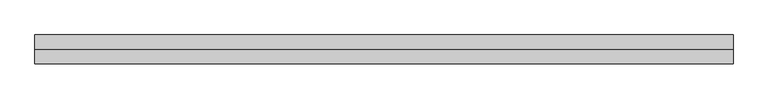
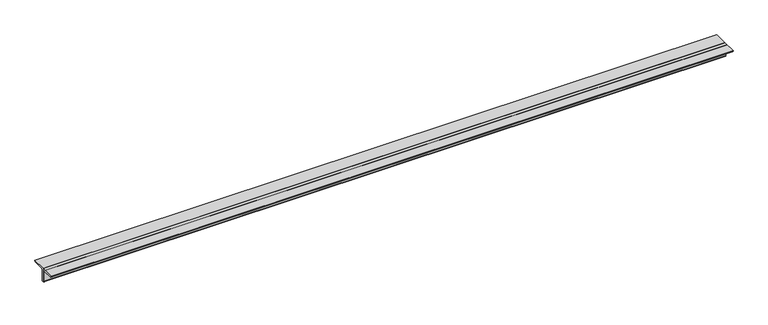
"""IFC4 building model written with IfcOpenShell, lengths in millimetres: member geometry, 0123_Steel Framing_2Ls-KSD3502 : H_SB_AR_S04_2Ls-130x130x12_VBR2."""

from ifc_helpers import new_model, si_unit, point, frame, frame_2d, origin, place, context, project, spatial, polyline, circle_curve, trimmed, segment, composite_curve, outline, extrude, source, transform, mapped, element, save


def member_81b2beba(model_context):
    return source(origin(), model_context, "Body", "SweptSolid", [
        extrude(outline(composite_curve([segment(polyline([(0.0, 36.4), (130.0, 36.4)]), True, "CONTINUOUS"), segment(trimmed(circle_curve(frame_2d((118.0, 36.4)), 12.0), [point((130.0, 36.4))], [point((118.0, 24.4))], False, "CARTESIAN"), True, "CONTINUOUS"), segment(polyline([(118.0, 24.4), (24.0, 24.4)]), True, "CONTINUOUS"), segment(trimmed(circle_curve(frame_2d((24.0, 12.4)), 12.0), [point((24.0, 24.4))], [point((12.0, 12.4))], True, "CARTESIAN"), True, "CONTINUOUS"), segment(polyline([(12.0, 12.4), (12.0, -81.6)]), True, "CONTINUOUS"), segment(trimmed(circle_curve(frame_2d((0.0, -81.6)), 12.0), [point((12.0, -81.6))], [point((0.0, -93.6))], False, "CARTESIAN"), True, "CONTINUOUS"), segment(polyline([(0.0, -93.6), (0.0, 36.4)]), True, "CONTINUOUS")], self_intersect=False)), frame((-3360.6041751, 0.0, 0.0), z_axis=(1.0, 0.0, 0.0), x_axis=(0.0, 1.0, 0.0)), (0.0, 0.0, 1.0), 6322.5847795),
        extrude(outline(composite_curve([segment(polyline([(0.0, 36.4), (0.0, -93.6)]), True, "CONTINUOUS"), segment(trimmed(circle_curve(frame_2d((0.0, -81.6)), 12.0), [point((0.0, -93.6))], [point((-12.0, -81.6))], False, "CARTESIAN"), True, "CONTINUOUS"), segment(polyline([(-12.0, -81.6), (-12.0, 12.4)]), True, "CONTINUOUS"), segment(trimmed(circle_curve(frame_2d((-24.0, 12.4)), 12.0), [point((-12.0, 12.4))], [point((-24.0, 24.4))], True, "CARTESIAN"), True, "CONTINUOUS"), segment(polyline([(-24.0, 24.4), (-118.0, 24.4)]), True, "CONTINUOUS"), segment(trimmed(circle_curve(frame_2d((-118.0, 36.4)), 12.0), [point((-118.0, 24.4))], [point((-130.0, 36.4))], False, "CARTESIAN"), True, "CONTINUOUS"), segment(polyline([(-130.0, 36.4), (0.0, 36.4)]), True, "CONTINUOUS")], self_intersect=False)), frame((-3360.6041751, 0.0, 0.0), z_axis=(1.0, 0.0, 0.0), x_axis=(0.0, 1.0, 0.0)), (0.0, 0.0, 1.0), 6322.5847795),
    ])


if __name__ == "__main__":
    model = new_model("IFC4")
    model_context = context("Model", 3, world=origin())
    ifc_project = project(units=[si_unit("LENGTHUNIT", "METRE", prefix="MILLI")], contexts=[model_context])
    site = spatial("IfcSite", under=ifc_project)
    building = spatial("IfcBuilding", under=site)
    placement = place(None, origin())
    member_shape = member_81b2beba(model_context)
    element("IfcMember", 1, ObjectType="0123_Steel Framing_2Ls-KSD3502 : H_SB_AR_S04_2Ls-130x130x12_VBR2", at=placement, inside=building, context=model_context, shape_type="MappedRepresentation", body=[
        mapped(member_shape, transform((0.0, 0.0, 0.0), x_axis=(1.0, 0.0, 0.0), y_axis=(0.0, 1.0, 0.0), z_axis=(0.0, 0.0, 1.0))),
    ])
    save(model, "model.ifc")

# Revit data of these elements
# Type "0123_Steel Framing_2Ls-KSD3502 : H_SB_AR_S04_2Ls-130x130x12_VBR2"
#   Assembly Code = "B10"
#   Legs = "SLBB"
#   W = 8.97
#   Perimeter = 1.04 m²/m
#   Nominal Weight = 46.80 kgf/m
#   Length [instance default] = 1000 mm
#   Space = 0 mm
#   b = 130 mm
#   d = 130 mm
#   t = 12 mm
#   y = 36.4 mm
#   A = 0.005952 m²
#   Structural Material [instance default] = Steel ASTM A36
# Element 1 (IfcMember, "0123_Steel Framing_2Ls-KSD3502 : H_SB_AR_S04_2Ls-130x130x12_VBR2")
#   Structural Material = Steel, 45-345
#   Materials on its faces: "Steel, 45-345"
# Materials
#   "Steel ASTM A36": class "Metal", colour RGB 199 199 199, transparency 0, Description = "Structural steel, ASTM A36 Grade B, mill finish", Cost = 0
#   "Steel, 45-345": class "Metal", colour RGB 189 187 185, transparency 0, Description = "Steel 345 MPa", Cost = 0
